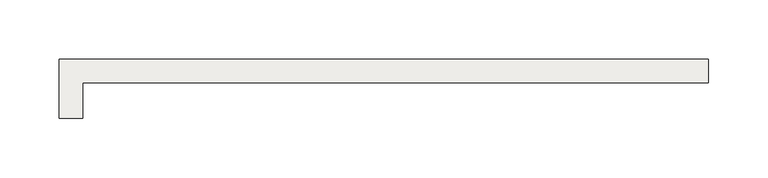
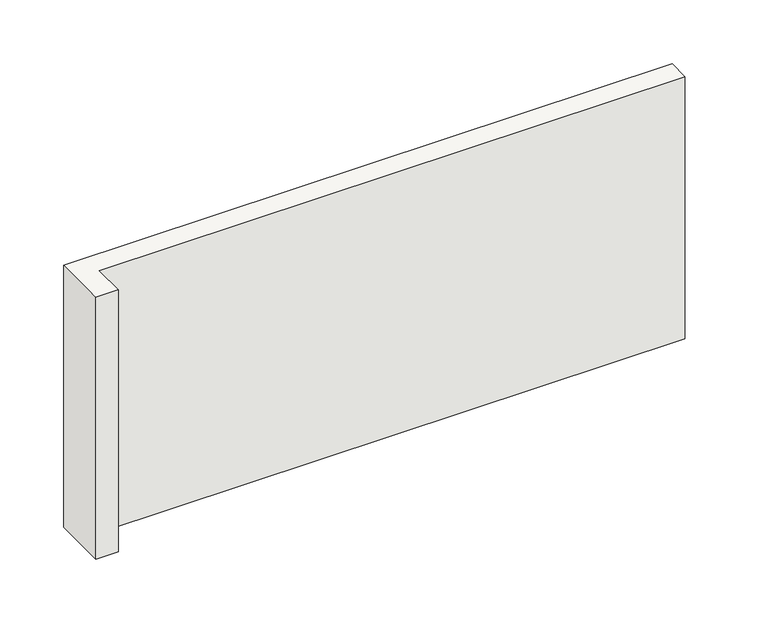
"""IFC4 building model written with IfcOpenShell, lengths in millimetres: slab geometry, FECHAMENTO DECK DE MADEIRA - PATAMAR ENTRADA 1 : FECHAMENTO DECK DE MADEIRA - PATAMAR ENTRADA 2."""

from ifc_helpers import new_model, si_unit, frame, origin, place, context, project, spatial, polyline, outline, extrude, source, transform, mapped, element, save


def slab_ac09833d(model_context):
    return source(origin(), model_context, "Body", "SweptSolid", [
        extrude(outline(polyline([(-7189.281307, -2045.5699847), (-7209.281307, -2045.5699847), (-7209.281307, -1995.5699847), (-6660.281307, -1995.5699847), (-6660.281307, -2015.5699847), (-7189.281307, -2015.5699847), (-7189.281307, -2045.5699847)])), frame((0.0, 0.0, 80.0), z_axis=(0.0, 0.0, 1.0), x_axis=(1.0, 0.0, 0.0)), (0.0, 0.0, 1.0), 250.0),
    ])


if __name__ == "__main__":
    model = new_model("IFC4")
    model_context = context("Model", 3, world=origin())
    ifc_project = project(units=[si_unit("LENGTHUNIT", "METRE", prefix="MILLI")], contexts=[model_context])
    site = spatial("IfcSite", under=ifc_project)
    building = spatial("IfcBuilding", under=site)
    placement = place(None, origin())
    slab_shape = slab_ac09833d(model_context)
    element("IfcSlab", 1, ObjectType="FECHAMENTO DECK DE MADEIRA - PATAMAR ENTRADA 1 : FECHAMENTO DECK DE MADEIRA - PATAMAR ENTRADA 2", at=placement, inside=building, context=model_context, shape_type="MappedRepresentation", body=[
        mapped(slab_shape, transform((0.0, 0.0, 0.0), x_axis=(1.0, 0.0, 0.0), y_axis=(0.0, 1.0, 0.0), z_axis=(0.0, 0.0, 1.0))),
    ])
    save(model, "model.ifc")

# Revit data of these elements
# Element 1 (IfcSlab, "FECHAMENTO DECK DE MADEIRA - PATAMAR ENTRADA 1 : FECHAMENTO DECK DE MADEIRA - PATAMAR ENTRADA 2")
#   Materials on its faces: ".DECK DE MADEIRA TRANSVERSAL"
# Materials
#   ".DECK DE MADEIRA TRANSVERSAL": class ".CC_MADEIRA REVEST.", colour RGB 169 114 85, transparency 0, Description = "Deck de madeira", Cost = 0
